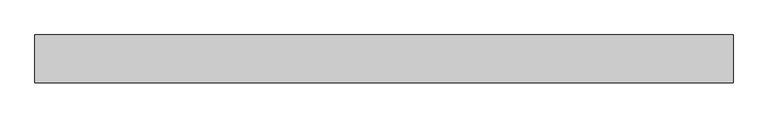
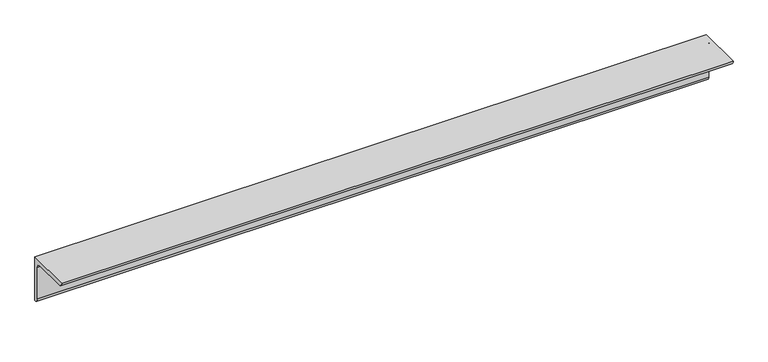
"""IFC4 building model written with IfcOpenShell, lengths in millimetres: member geometry, 0912_Steel Framing_L-KSD3502 : H_SB_AR_S03_L-130x130x12_HBR3."""

from ifc_helpers import new_model, si_unit, point, frame, frame_2d, origin, place, context, project, spatial, polyline, circle_curve, trimmed, segment, composite_curve, outline, extrude, source, transform, mapped, element, save


def member_5231fe44(model_context):
    return source(origin(), model_context, "Body", "SweptSolid", [
        extrude(outline(composite_curve([segment(polyline([(36.4, 36.4), (36.4, -93.6)]), True, "CONTINUOUS"), segment(trimmed(circle_curve(frame_2d((36.4, -81.6)), 12.0), [point((36.4, -93.6))], [point((24.4, -81.6))], False, "CARTESIAN"), True, "CONTINUOUS"), segment(polyline([(24.4, -81.6), (24.4, 12.4)]), True, "CONTINUOUS"), segment(trimmed(circle_curve(frame_2d((12.4, 12.4)), 12.0), [point((24.4, 12.4))], [point((12.4, 24.4))], True, "CARTESIAN"), True, "CONTINUOUS"), segment(polyline([(12.4, 24.4), (-81.6, 24.4)]), True, "CONTINUOUS"), segment(trimmed(circle_curve(frame_2d((-81.6, 36.4)), 12.0), [point((-81.6, 24.4))], [point((-93.6, 36.4))], False, "CARTESIAN"), True, "CONTINUOUS"), segment(polyline([(-93.6, 36.4), (36.4, 36.4)]), True, "CONTINUOUS")], self_intersect=False)), frame((-1004.5243078, 0.0, 0.0), z_axis=(1.0, 0.0, 0.0), x_axis=(0.0, 1.0, 0.0)), (0.0, 0.0, 1.0), 1889.881949),
    ])


if __name__ == "__main__":
    model = new_model("IFC4")
    model_context = context("Model", 3, world=origin())
    ifc_project = project(units=[si_unit("LENGTHUNIT", "METRE", prefix="MILLI")], contexts=[model_context])
    site = spatial("IfcSite", under=ifc_project)
    building = spatial("IfcBuilding", under=site)
    placement = place(None, origin())
    member_shape = member_5231fe44(model_context)
    element("IfcMember", 1, ObjectType="0912_Steel Framing_L-KSD3502 : H_SB_AR_S03_L-130x130x12_HBR3", at=placement, inside=building, context=model_context, shape_type="MappedRepresentation", body=[
        mapped(member_shape, transform((0.0, 0.0, 0.0), x_axis=(1.0, 0.0, 0.0), y_axis=(0.0, 1.0, 0.0), z_axis=(0.0, 0.0, 1.0))),
    ])
    save(model, "model.ifc")

# Revit data of these elements
# Type "0912_Steel Framing_L-KSD3502 : H_SB_AR_S03_L-130x130x12_HBR3"
#   k = 25 mm
#   Perimeter = 0.52 m²/m
#   Nominal Weight = 23.40 kgf/m
#   Length [instance default] = 1000 mm
#   b = 130 mm
#   d = 130 mm
#   t = 12 mm
#   x = 36.4 mm
#   y = 36.4 mm
#   A = 2976.00 m²
#   Structural Material [instance default] = Steel, 45-345
# Element 1 (IfcMember, "0912_Steel Framing_L-KSD3502 : H_SB_AR_S03_L-130x130x12_HBR3")
#   Structural Material = Steel ASTM A36
#   Materials on its faces: "Steel ASTM A36"
# Materials
#   "Steel, 45-345": class "Metal", colour RGB 189 187 185, transparency 0, Description = "Steel 345 MPa", Cost = 0
#   "Steel ASTM A36": class "Metal", colour RGB 199 199 199, transparency 0, Description = "Structural steel, ASTM A36 Grade B, mill finish", Cost = 0
